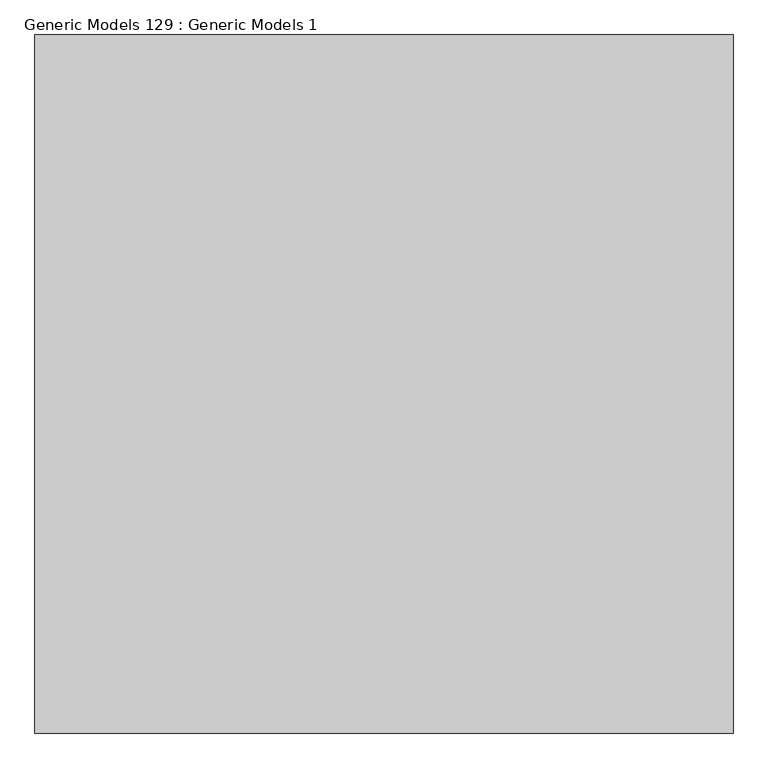
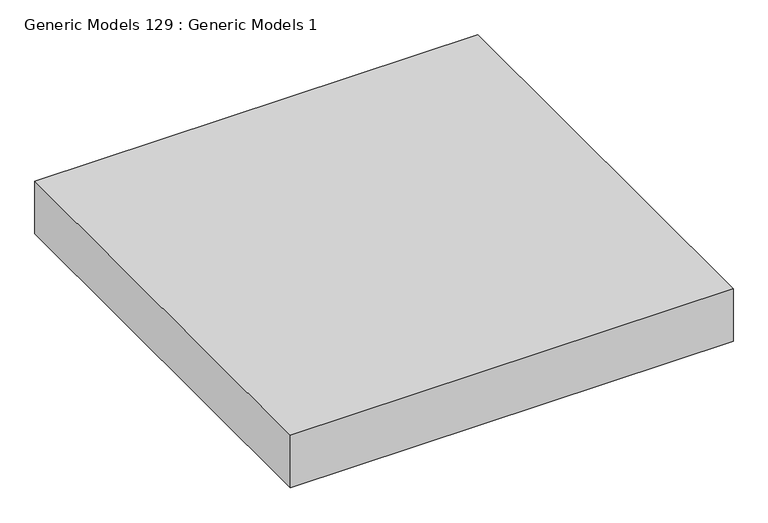
"""IFC4 building model written with IfcOpenShell, lengths in millimetres: proxy geometry, Generic Models 129 : Generic Models 1."""

from ifc_helpers import new_model, si_unit, frame, origin, place, context, project, spatial, polyline, outline, extrude, source, transform, mapped, element, save


def generic_models_129_generic_models_1_8999e842(model_context):
    return source(origin(), model_context, "Body", "SweptSolid", [
        extrude(outline(polyline([(47499.4360531, 0.0), (46280.2360531, 0.0), (46280.2360531, 1219.2), (47499.4360531, 1219.2), (47499.4360531, 0.0)])), frame((0.0, 0.0, -378.376067), z_axis=(0.0, 0.0, 1.0), x_axis=(1.0, 0.0, 0.0)), (0.0, 0.0, 1.0), 152.4),
    ])


if __name__ == "__main__":
    model = new_model("IFC4")
    model_context = context("Model", 3, world=origin())
    ifc_project = project(units=[si_unit("LENGTHUNIT", "METRE", prefix="MILLI")], contexts=[model_context])
    site = spatial("IfcSite", under=ifc_project)
    building = spatial("IfcBuilding", under=site)
    placement = place(None, origin())
    generic_models_129_generic_models_1_shape = generic_models_129_generic_models_1_8999e842(model_context)
    element("IfcBuildingElementProxy", 1, Name="Generic Models 129 : Generic Models 1", ObjectType="Generic Models 129 : Generic Models 1", at=placement, inside=building, context=model_context, shape_type="MappedRepresentation", body=[
        mapped(generic_models_129_generic_models_1_shape, transform((0.0, 0.0, 0.0), x_axis=(1.0, 0.0, 0.0), y_axis=(0.0, 1.0, 0.0), z_axis=(0.0, 0.0, 1.0))),
    ])
    save(model, "model.ifc")

# Revit data of these elements
# Element 1 (IfcBuildingElementProxy, "Generic Models 129 : Generic Models 1")
#   Materials on its faces: "EXISTING SLAB"
# Materials
#   "EXISTING SLAB": class "Concrete", colour RGB 129 132 118, transparency 0, Description = "Lightweight concrete", Cost = 0
